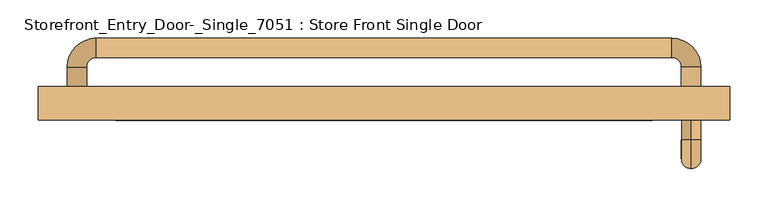
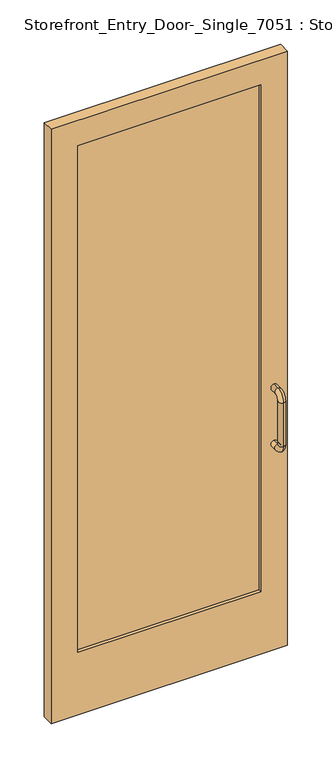
"""IFC4 building model written with IfcOpenShell, lengths in millimetres: door geometry, Storefront_Entry_Door-_Single_7051 : Store Front Single Door."""

import ifcopenshell
import ifcopenshell.guid

model = None  # the IFC model being written
_history = None  # IfcOwnerHistory: only IFC2X3 demands one
_inside = {}  # id of a spatial element -> (the spatial element, [elements in it])
_under = {}  # id of a project, library or spatial element -> (it, [spatial elements below it])
_declared = {}  # id of a project -> (the project, [libraries it declares])
_typed = {}  # id of a type object -> (the type object, [elements of that type])
_made_of = {}  # id of a material, layer set ... -> (it, [elements and type objects made of it])


def new_model(schema):
    """Start an empty IFC model of exactly this schema.

    Asked for "IFC4X3", IfcOpenShell would pick the latest addendum, in which some entities
    have other attributes; the version numbers below select the first issue.
    IFC2X3 requires an IfcOwnerHistory on every rooted entity: one is made here for all.
    """
    global model, _history
    if schema == "IFC4X3":
        model = ifcopenshell.file(schema_version=(4, 3, 0, 0))
    else:
        model = ifcopenshell.file(schema=schema)
    _inside.clear()
    _under.clear()
    _declared.clear()
    _typed.clear()
    _made_of.clear()
    _history = None
    if model.schema == "IFC2X3":
        org = make("IfcOrganization", Name="unknown")
        user = make(
            "IfcPersonAndOrganization",
            ThePerson=make("IfcPerson", FamilyName="unknown"),
            TheOrganization=org,
        )
        app = make(
            "IfcApplication",
            ApplicationDeveloper=org,
            Version="unknown",
            ApplicationFullName="unknown",
            ApplicationIdentifier="unknown",
        )
        _history = make(
            "IfcOwnerHistory",
            OwningUser=user,
            OwningApplication=app,
            ChangeAction="ADDED",
            CreationDate=0,
        )
    return model


def make(cls, **values):
    """One entity of the class cls with the attributes given. An attribute that is None is left unset."""
    return model.create_entity(
        cls, **{name: value for name, value in values.items() if value is not None}
    )


def rooted(cls, **values):
    """An entity with a GlobalId (a new one), such as an element, a storey or a relation."""
    return make(cls, GlobalId=ifcopenshell.guid.new(), OwnerHistory=_history, **values)


def si_unit(unit_type, name, prefix=None):
    """IfcSIUnit, for example si_unit("LENGTHUNIT", "METRE", prefix="MILLI")."""
    return make("IfcSIUnit", UnitType=unit_type, Prefix=prefix, Name=name)


def assignment(units):
    """IfcUnitAssignment: the units of a project."""
    return None if units is None else make("IfcUnitAssignment", Units=units)


def point(xyz):
    """IfcCartesianPoint."""
    return None if xyz is None else make("IfcCartesianPoint", Coordinates=xyz)


def direction(xyz):
    """IfcDirection."""
    return None if xyz is None else make("IfcDirection", DirectionRatios=xyz)


def frame(location, z_axis=None, x_axis=None):
    """IfcAxis2Placement3D, a coordinate frame: its origin and axes. An axis left out is left unset."""
    return make(
        "IfcAxis2Placement3D",
        Location=point(location),
        Axis=direction(z_axis),
        RefDirection=direction(x_axis),
    )


def origin():
    """The frame at (0, 0, 0) with its axes left unset."""
    return frame((0.0, 0.0, 0.0))


def place(relative_to, where):
    """IfcLocalPlacement: puts the frame where relative to a parent placement (None: the world)."""
    return make(
        "IfcLocalPlacement", PlacementRelTo=relative_to, RelativePlacement=where
    )


def context(
    kind, dimensions, precision=None, world=None, true_north=None, identifier=None
):
    """IfcGeometricRepresentationContext, for example the 3D "Model" context."""
    return make(
        "IfcGeometricRepresentationContext",
        ContextIdentifier=identifier,
        ContextType=kind,
        CoordinateSpaceDimension=dimensions,
        Precision=precision,
        WorldCoordinateSystem=world,
        TrueNorth=true_north,
    )


def project(units=None, contexts=None):
    """IfcProject with its units and contexts."""
    return rooted(
        "IfcProject",
        Name="project",
        RepresentationContexts=contexts,
        UnitsInContext=assignment(units),
    )


def spatial(cls, under=None, at=None, **own):
    """A site, building, storey or space (cls), placed at a placement, below another one or the project."""
    s = rooted(cls, ObjectPlacement=at, **own)
    if under is not None:
        _under.setdefault(under.id(), (under, []))[1].append(s)
    return s


def polyline(points):
    """IfcPolyline through the points."""
    return make("IfcPolyline", Points=[point(p) for p in points])


def circle_curve(where, radius):
    """IfcCircle in the frame where."""
    return make("IfcCircle", Position=where, Radius=radius)


def ellipse_curve(where, semi_axis1, semi_axis2):
    """IfcEllipse in the frame where."""
    return make(
        "IfcEllipse", Position=where, SemiAxis1=semi_axis1, SemiAxis2=semi_axis2
    )


def trimmed(basis, trim1, trim2, sense, master):
    """IfcTrimmedCurve: the piece of a basis curve between two trims."""
    return make(
        "IfcTrimmedCurve",
        BasisCurve=basis,
        Trim1=trim1,
        Trim2=trim2,
        SenseAgreement=sense,
        MasterRepresentation=master,
    )


def outline(outer, holes=None, kind="AREA"):
    """IfcArbitraryClosedProfileDef: a profile drawn as a closed curve; with holes, ...WithVoids."""
    if holes is None:
        return make("IfcArbitraryClosedProfileDef", ProfileType=kind, OuterCurve=outer)
    return make(
        "IfcArbitraryProfileDefWithVoids",
        ProfileType=kind,
        OuterCurve=outer,
        InnerCurves=holes,
    )


def extrude(swept, where, along, depth):
    """IfcExtrudedAreaSolid: the profile swept, set in the frame where, extruded along a direction by depth."""
    return make(
        "IfcExtrudedAreaSolid",
        SweptArea=swept,
        Position=where,
        ExtrudedDirection=direction(along),
        Depth=depth,
    )


def shape(context_of_items, identifier, shape_type, items):
    """IfcShapeRepresentation: the items that make up one representation, for example the "Body"."""
    return make(
        "IfcShapeRepresentation",
        ContextOfItems=context_of_items,
        RepresentationIdentifier=identifier,
        RepresentationType=shape_type,
        Items=items,
    )


def source(mapping_origin, context_of_items, identifier, shape_type, items):
    """IfcRepresentationMap: a shape defined once, which mapped items show again and again."""
    return make(
        "IfcRepresentationMap",
        MappingOrigin=mapping_origin,
        MappedRepresentation=shape(context_of_items, identifier, shape_type, items),
    )


def transform(
    local_origin,
    x_axis=None,
    y_axis=None,
    z_axis=None,
    scale=None,
    scale2=None,
    scale3=None,
    uniform=True,
):
    """IfcCartesianTransformationOperator3D, or its non-uniform kind. x_axis, y_axis, z_axis: its Axis1, 2, 3."""
    if uniform:
        return make(
            "IfcCartesianTransformationOperator3D",
            Axis1=direction(x_axis),
            Axis2=direction(y_axis),
            LocalOrigin=point(local_origin),
            Scale=scale,
            Axis3=direction(z_axis),
        )
    return make(
        "IfcCartesianTransformationOperator3DnonUniform",
        Axis1=direction(x_axis),
        Axis2=direction(y_axis),
        LocalOrigin=point(local_origin),
        Scale=scale,
        Axis3=direction(z_axis),
        Scale2=scale2,
        Scale3=scale3,
    )


def mapped(mapping_source, mapping_target):
    """IfcMappedItem: shows the shape of a source again, moved by a transform."""
    return make(
        "IfcMappedItem", MappingSource=mapping_source, MappingTarget=mapping_target
    )


def made_of(thing, what):
    """Note that an element or type object is made of a material, layer set ...; save() writes the relation."""
    if what is not None:
        _made_of.setdefault(what.id(), (what, []))[1].append(thing)
    return thing


def element(
    cls,
    number,
    at=None,
    inside=None,
    cuts=None,
    type_object=None,
    material=None,
    context=None,
    identifier="Body",
    shape_type=None,
    held_by="IfcProductDefinitionShape",
    body=None,
    shapes=None,
    **own,
):
    """One element of the class cls, such as IfcWall. Its Tag is "e" and its number.

    at: its placement. inside: the storey or other place that contains it. cuts: it is an
    opening in that element (IfcRelVoidsElement). A single representation is given by context,
    identifier, shape_type and body (its items); several are given by shapes. held_by: the class
    of the entity that holds the representations. save() writes the other relations.
    """
    e = rooted(cls, Tag="e%d" % number, ObjectPlacement=at, **own)
    if body is not None:
        shapes = [shape(context, identifier, shape_type, body)]
    if shapes is not None:
        e.Representation = make(held_by, Representations=shapes)
    if inside is not None:
        _inside.setdefault(inside.id(), (inside, []))[1].append(e)
    if cuts is not None:
        rooted(
            "IfcRelVoidsElement", RelatingBuildingElement=cuts, RelatedOpeningElement=e
        )
    if type_object is not None:
        _typed.setdefault(type_object.id(), (type_object, []))[1].append(e)
    return made_of(e, material)


def aggregate(whole, parts):
    """IfcRelAggregates: a whole, such as a stair, and the parts it consists of."""
    return rooted("IfcRelAggregates", RelatingObject=whole, RelatedObjects=parts)


def save(model, path):
    """Write the relations noted so far, then the file.

    IfcRelAggregates (storeys below a building ...), IfcRelContainedInSpatialStructure (elements
    in a storey), IfcRelDefinesByType, IfcRelAssociatesMaterial and IfcRelDeclares: one each for
    every whole, place, type object, material and project.
    """
    for whole, parts in _under.values():
        aggregate(whole, parts)
    for where, things in _inside.values():
        rooted(
            "IfcRelContainedInSpatialStructure",
            RelatedElements=things,
            RelatingStructure=where,
        )
    for kind, things in _typed.values():
        rooted("IfcRelDefinesByType", RelatedObjects=things, RelatingType=kind)
    for what, things in _made_of.values():
        rooted("IfcRelAssociatesMaterial", RelatedObjects=things, RelatingMaterial=what)
    for by, libraries in _declared.values():
        rooted("IfcRelDeclares", RelatingContext=by, RelatedDefinitions=libraries)
    model.write(path)


def plane_surface(at):
    """IfcPlane: the flat surface through the origin of the frame at, square to its z axis."""
    return make("IfcPlane", Position=at)


def cylinder_surface(at, radius):
    """IfcCylindricalSurface: all points at the distance radius from the z axis of the frame at."""
    return make("IfcCylindricalSurface", Position=at, Radius=radius)


def revolved_surface(curve, axis_point, axis_direction):
    """IfcSurfaceOfRevolution: the curve turned about the line through axis_point along axis_direction."""
    return make(
        "IfcSurfaceOfRevolution",
        SweptCurve=make("IfcArbitraryOpenProfileDef", ProfileType="CURVE", Curve=curve),
        AxisPosition=make("IfcAxis1Placement", Location=point(axis_point), Axis=direction(axis_direction)),
    )


def advanced_brep(points, edges, surfaces, faces):
    """IfcAdvancedBrep: a solid bounded by faces that lie on surfaces and meet in shared edges.

    An edge is (start, end): straight between two places in points (the first is 0);
    or (start, end, curve); or (start, end, curve, False) where it runs against its curve.
    A face is (place in surfaces, loops), or (place, loops, False) where it looks against
    its surface's normal. A loop lists edges by number (the first is 1), with a minus sign
    where the edge is run from its end to its start. The first loop is the outer one.
    """
    corners = [point(p) for p in points]
    vertices = [make("IfcVertexPoint", VertexGeometry=c) for c in corners]
    made = []
    for start, end, *more in edges:
        made.append(
            make(
                "IfcEdgeCurve",
                EdgeStart=vertices[start],
                EdgeEnd=vertices[end],
                EdgeGeometry=more[0] if more else make("IfcPolyline", Points=[corners[start], corners[end]]),
                SameSense=more[1] if len(more) > 1 else True,
            )
        )
    hull = []
    for where, loops, *sense in faces:
        bounds = []
        for j, loop in enumerate(loops):
            ring = [make("IfcOrientedEdge", EdgeElement=made[abs(k) - 1], Orientation=k > 0) for k in loop]
            bounds.append(
                make(
                    "IfcFaceOuterBound" if j == 0 else "IfcFaceBound",
                    Bound=make("IfcEdgeLoop", EdgeList=ring),
                    Orientation=True,
                )
            )
        hull.append(make("IfcAdvancedFace", Bounds=bounds, FaceSurface=surfaces[where], SameSense=sense[0] if sense else True))
    return make("IfcAdvancedBrep", Outer=make("IfcClosedShell", CfsFaces=hull))


def storefront_entry_door_single_7051_store_front_single_door_ff742114(model_context):
    return source(origin(), model_context, "Body", "SolidModel", [
        advanced_brep(
        [(402.7714285, -50.8, 1054.1), (402.7714285, -50.8, 1079.5), (402.7714285, -76.2, 1079.5), (402.7714285, -76.2, 1054.1), (402.7714285, -114.3, 1041.4), (402.7714285, -88.9, 1041.4), (402.7714285, -114.3, 863.6), (402.7714285, -88.9, 863.6), (402.7714285, -76.2, 825.5), (402.7714285, -76.2, 850.9), (402.7714285, -50.8, 850.9), (402.7714285, -50.8, 825.5)],
        [
            (0, 1, circle_curve(frame((402.7714285, -50.8, 1066.8), z_axis=(0.0, 1.0, 0.0), x_axis=(0.0, 0.0, 1.0)), 12.7)),
            (1, 0, circle_curve(frame((402.7714285, -50.8, 1066.8), z_axis=(0.0, 1.0, 0.0), x_axis=(0.0, 0.0, 1.0)), 12.7)),
            (1, 2),
            (2, 3, circle_curve(frame((402.7714285, -76.2, 1066.8), z_axis=(0.0, 1.0, 0.0), x_axis=(0.0, 0.0, 1.0)), 12.7)),
            (3, 0),
            (3, 2, circle_curve(frame((402.7714285, -76.2, 1066.8), z_axis=(0.0, 1.0, 0.0), x_axis=(0.0, 0.0, 1.0)), 12.7)),
            (4, 5, circle_curve(frame((402.7714285, -101.6, 1041.4), z_axis=(0.0, 0.0, 1.0), x_axis=(0.0, -1.0, 0.0)), 12.7)),
            (5, 3, circle_curve(frame((402.7714285, -76.2, 1041.4), z_axis=(-1.0, 0.0, 0.0), x_axis=(0.0, 0.0, 1.0)), 12.7)),
            (2, 4, circle_curve(frame((402.7714285, -76.2, 1041.4), z_axis=(1.0, 0.0, 0.0), x_axis=(0.0, 0.0, 1.0)), 38.1)),
            (5, 4, circle_curve(frame((402.7714285, -101.6, 1041.4), z_axis=(0.0, 0.0, 1.0), x_axis=(0.0, -1.0, 0.0)), 12.7)),
            (4, 6),
            (6, 7, circle_curve(frame((402.7714285, -101.6, 863.6), z_axis=(0.0, 0.0, 1.0), x_axis=(0.0, -1.0, 0.0)), 12.7)),
            (7, 5),
            (7, 6, circle_curve(frame((402.7714285, -101.6, 863.6), z_axis=(0.0, 0.0, 1.0), x_axis=(0.0, -1.0, 0.0)), 12.7)),
            (8, 9, circle_curve(frame((402.7714285, -76.2, 838.2), z_axis=(0.0, -1.0, 0.0), x_axis=(0.0, 0.0, -1.0)), 12.7)),
            (9, 7, circle_curve(frame((402.7714285, -76.2, 863.6), z_axis=(-1.0, 0.0, 0.0), x_axis=(0.0, -1.0, 0.0)), 12.7)),
            (6, 8, circle_curve(frame((402.7714285, -76.2, 863.6), z_axis=(1.0, 0.0, 0.0), x_axis=(0.0, -1.0, 0.0)), 38.1)),
            (9, 8, circle_curve(frame((402.7714285, -76.2, 838.2), z_axis=(0.0, -1.0, 0.0), x_axis=(0.0, 0.0, -1.0)), 12.7)),
            (10, 11, circle_curve(frame((402.7714285, -50.8, 838.2), z_axis=(0.0, 1.0, 0.0), x_axis=(0.0, 0.0, -1.0)), 12.7)),
            (11, 10, circle_curve(frame((402.7714285, -50.8, 838.2), z_axis=(0.0, 1.0, 0.0), x_axis=(0.0, 0.0, -1.0)), 12.7)),
            (8, 11),
            (10, 9),
        ],
        [
            plane_surface(frame((402.7714285, -50.8, 1066.8), z_axis=(0.0, 1.0, 0.0), x_axis=(1.0, 0.0, 0.0))),
            cylinder_surface(frame((402.7714285, -50.8, 1066.8), z_axis=(0.0, 1.0, 0.0), x_axis=(0.0, 0.0, 1.0)), 12.7),
            revolved_surface(trimmed(ellipse_curve(frame((402.7714285, -76.2, 1066.8), z_axis=(0.0, -1.0, 0.0), x_axis=(0.0, 0.0, 1.0)), 12.7, 12.7), [point((402.7714285, -76.2, 1054.1))], [point((402.7714285, -76.2, 1079.5))], True, "CARTESIAN"), (402.7714285, -76.2, 1041.4), (-1.0, 0.0, 0.0)),
            revolved_surface(trimmed(ellipse_curve(frame((402.7714285, -76.2, 1066.8), z_axis=(0.0, -1.0, 0.0), x_axis=(0.0, 0.0, 1.0)), 12.7, 12.7), [point((402.7714285, -76.2, 1079.5))], [point((402.7714285, -76.2, 1054.1))], True, "CARTESIAN"), (402.7714285, -76.2, 1041.4), (-1.0, 0.0, 0.0)),
            cylinder_surface(frame((402.7714285, -101.6, 1041.4), z_axis=(0.0, 0.0, 1.0), x_axis=(0.0, -1.0, 0.0)), 12.7),
            revolved_surface(trimmed(ellipse_curve(frame((402.7714285, -101.6, 863.6), z_axis=(0.0, 0.0, -1.0), x_axis=(0.0, -1.0, 0.0)), 12.7, 12.7), [point((402.7714285, -88.9, 863.6))], [point((402.7714285, -114.3, 863.6))], True, "CARTESIAN"), (402.7714285, -76.2, 863.6), (-1.0, 0.0, 0.0)),
            revolved_surface(trimmed(ellipse_curve(frame((402.7714285, -101.6, 863.6), z_axis=(0.0, 0.0, -1.0), x_axis=(0.0, -1.0, 0.0)), 12.7, 12.7), [point((402.7714285, -114.3, 863.6))], [point((402.7714285, -88.9, 863.6))], True, "CARTESIAN"), (402.7714285, -76.2, 863.6), (-1.0, 0.0, 0.0)),
            plane_surface(frame((402.7714285, -50.8, 838.2), z_axis=(0.0, 1.0, 0.0), x_axis=(1.0, 0.0, 0.0))),
            cylinder_surface(frame((402.7714285, -76.2, 838.2), z_axis=(0.0, -1.0, 0.0), x_axis=(0.0, 0.0, -1.0)), 12.7),
        ],
        [
            (0, [[1, 2]]),
            (1, [[3, 4, 5, -2]]),
            (1, [[-5, 6, -3, -1]]),
            (2, [[7, 8, -4, 9]]),
            (3, [[10, -9, -6, -8]]),
            (4, [[11, 12, 13, -7]]),
            (4, [[-13, 14, -11, -10]]),
            (5, [[15, 16, -12, 17]]),
            (6, [[18, -17, -14, -16]]),
            (7, [[19, 20]]),
            (8, [[21, -19, 22, -15]]),
            (8, [[-22, -20, -21, -18]]),
        ],
    ),
        advanced_brep(
        [(390.0714285, -6.35, 1066.8), (415.4714285, -6.35, 1066.8), (415.4714285, 19.05, 1066.8), (390.0714285, 19.05, 1066.8), (377.3714285, 57.15, 1066.8), (377.3714285, 31.75, 1066.8), (-377.3714285, 57.15, 1066.8), (-377.3714285, 31.75, 1066.8), (-415.4714285, 19.05, 1066.8), (-390.0714285, 19.05, 1066.8), (-390.0714285, -6.35, 1066.8), (-415.4714285, -6.35, 1066.8)],
        [
            (0, 1, circle_curve(frame((402.7714285, -6.35, 1066.8), z_axis=(0.0, -1.0, 0.0), x_axis=(1.0, 0.0, 0.0)), 12.7)),
            (1, 0, circle_curve(frame((402.7714285, -6.35, 1066.8), z_axis=(0.0, -1.0, 0.0), x_axis=(1.0, 0.0, 0.0)), 12.7)),
            (1, 2),
            (2, 3, circle_curve(frame((402.7714285, 19.05, 1066.8), z_axis=(0.0, -1.0, 0.0), x_axis=(1.0, 0.0, 0.0)), 12.7)),
            (3, 0),
            (3, 2, circle_curve(frame((402.7714285, 19.05, 1066.8), z_axis=(0.0, -1.0, 0.0), x_axis=(1.0, 0.0, 0.0)), 12.7)),
            (4, 5, circle_curve(frame((377.3714285, 44.45, 1066.8), z_axis=(1.0, 0.0, 0.0), x_axis=(0.0, 1.0, 0.0)), 12.7)),
            (5, 3, circle_curve(frame((377.3714285, 19.05, 1066.8), z_axis=(0.0, 0.0, -1.0), x_axis=(1.0, 0.0, 0.0)), 12.7)),
            (2, 4, circle_curve(frame((377.3714285, 19.05, 1066.8), z_axis=(0.0, 0.0, 1.0), x_axis=(1.0, 0.0, 0.0)), 38.1)),
            (5, 4, circle_curve(frame((377.3714285, 44.45, 1066.8), z_axis=(1.0, 0.0, 0.0), x_axis=(0.0, 1.0, 0.0)), 12.7)),
            (4, 6),
            (6, 7, circle_curve(frame((-377.3714285, 44.45, 1066.8), z_axis=(1.0, 0.0, 0.0), x_axis=(0.0, 1.0, 0.0)), 12.7)),
            (7, 5),
            (7, 6, circle_curve(frame((-377.3714285, 44.45, 1066.8), z_axis=(1.0, 0.0, 0.0), x_axis=(0.0, 1.0, 0.0)), 12.7)),
            (8, 9, circle_curve(frame((-402.7714285, 19.05, 1066.8), z_axis=(0.0, 1.0, 0.0), x_axis=(-1.0, 0.0, 0.0)), 12.7)),
            (9, 7, circle_curve(frame((-377.3714285, 19.05, 1066.8), z_axis=(0.0, 0.0, -1.0), x_axis=(0.0, 1.0, 0.0)), 12.7)),
            (6, 8, circle_curve(frame((-377.3714285, 19.05, 1066.8), z_axis=(0.0, 0.0, 1.0), x_axis=(0.0, 1.0, 0.0)), 38.1)),
            (9, 8, circle_curve(frame((-402.7714285, 19.05, 1066.8), z_axis=(0.0, 1.0, 0.0), x_axis=(-1.0, 0.0, 0.0)), 12.7)),
            (10, 11, circle_curve(frame((-402.7714285, -6.35, 1066.8), z_axis=(0.0, -1.0, 0.0), x_axis=(-1.0, 0.0, 0.0)), 12.7)),
            (11, 10, circle_curve(frame((-402.7714285, -6.35, 1066.8), z_axis=(0.0, -1.0, 0.0), x_axis=(-1.0, 0.0, 0.0)), 12.7)),
            (8, 11),
            (10, 9),
        ],
        [
            plane_surface(frame((402.7714285, -6.35, 1066.8), z_axis=(0.0, -1.0, 0.0), x_axis=(0.0, 0.0, 1.0))),
            cylinder_surface(frame((402.7714285, -6.35, 1066.8), z_axis=(0.0, -1.0, 0.0), x_axis=(1.0, 0.0, 0.0)), 12.7),
            revolved_surface(trimmed(ellipse_curve(frame((402.7714285, 19.05, 1066.8), z_axis=(0.0, 1.0, 0.0), x_axis=(1.0, 0.0, 0.0)), 12.7, 12.7), [point((390.0714285, 19.05, 1066.8))], [point((415.4714285, 19.05, 1066.8))], True, "CARTESIAN"), (377.3714285, 19.05, 1066.8), (0.0, 0.0, -1.0)),
            revolved_surface(trimmed(ellipse_curve(frame((402.7714285, 19.05, 1066.8), z_axis=(0.0, 1.0, 0.0), x_axis=(1.0, 0.0, 0.0)), 12.7, 12.7), [point((415.4714285, 19.05, 1066.8))], [point((390.0714285, 19.05, 1066.8))], True, "CARTESIAN"), (377.3714285, 19.05, 1066.8), (0.0, 0.0, -1.0)),
            cylinder_surface(frame((377.3714285, 44.45, 1066.8), z_axis=(1.0, 0.0, 0.0), x_axis=(0.0, 1.0, 0.0)), 12.7),
            revolved_surface(trimmed(ellipse_curve(frame((-377.3714285, 44.45, 1066.8), z_axis=(-1.0, 0.0, 0.0), x_axis=(0.0, 1.0, 0.0)), 12.7, 12.7), [point((-377.3714285, 31.75, 1066.8))], [point((-377.3714285, 57.15, 1066.8))], True, "CARTESIAN"), (-377.3714285, 19.05, 1066.8), (0.0, 0.0, -1.0)),
            revolved_surface(trimmed(ellipse_curve(frame((-377.3714285, 44.45, 1066.8), z_axis=(-1.0, 0.0, 0.0), x_axis=(0.0, 1.0, 0.0)), 12.7, 12.7), [point((-377.3714285, 57.15, 1066.8))], [point((-377.3714285, 31.75, 1066.8))], True, "CARTESIAN"), (-377.3714285, 19.05, 1066.8), (0.0, 0.0, -1.0)),
            plane_surface(frame((-402.7714285, -6.35, 1066.8), z_axis=(0.0, -1.0, 0.0), x_axis=(0.0, 0.0, 1.0))),
            cylinder_surface(frame((-402.7714285, 19.05, 1066.8), z_axis=(0.0, 1.0, 0.0), x_axis=(-1.0, 0.0, 0.0)), 12.7),
        ],
        [
            (0, [[1, 2]]),
            (1, [[3, 4, 5, -2]]),
            (1, [[-5, 6, -3, -1]]),
            (2, [[7, 8, -4, 9]]),
            (3, [[10, -9, -6, -8]]),
            (4, [[11, 12, 13, -7]]),
            (4, [[-13, 14, -11, -10]]),
            (5, [[15, 16, -12, 17]]),
            (6, [[18, -17, -14, -16]]),
            (7, [[19, 20]]),
            (8, [[21, -19, 22, -15]]),
            (8, [[-22, -20, -21, -18]]),
        ],
    ),
        extrude(outline(polyline([(351.9714285, -19.05), (351.9714285, -38.1), (-351.9714285, -38.1), (-351.9714285, -19.05), (351.9714285, -19.05)])), frame((0.0, 0.0, 254.0), z_axis=(0.0, 0.0, 1.0), x_axis=(1.0, 0.0, 0.0)), (0.0, 0.0, 1.0), 2057.4),
        extrude(outline(polyline([(2413.0, 453.5714285), (2413.0, -453.5714285), (0.0, -453.5714285), (0.0, 453.5714285), (2413.0, 453.5714285)]), holes=[polyline([(2311.4, -351.9714285), (2311.4, 351.9714285), (254.0, 351.9714285), (254.0, -351.9714285), (2311.4, -351.9714285)])]), frame((0.0, -50.8, 0.0), z_axis=(0.0, 1.0, 0.0), x_axis=(0.0, 0.0, 1.0)), (0.0, 0.0, 1.0), 44.45),
    ])


if __name__ == "__main__":
    model = new_model("IFC4")
    model_context = context("Model", 3, world=origin())
    ifc_project = project(units=[si_unit("LENGTHUNIT", "METRE", prefix="MILLI")], contexts=[model_context])
    site = spatial("IfcSite", under=ifc_project)
    building = spatial("IfcBuilding", under=site)
    placement = place(None, origin())
    storefront_entry_door_single_7051_store_front_single_door_shape = storefront_entry_door_single_7051_store_front_single_door_ff742114(model_context)
    element("IfcDoor", 1, ObjectType="Storefront_Entry_Door-_Single_7051 : Store Front Single Door", at=placement, inside=building, context=model_context, shape_type="MappedRepresentation", body=[
        mapped(storefront_entry_door_single_7051_store_front_single_door_shape, transform((0.0, 0.0, 0.0), x_axis=(1.0, 0.0, 0.0), y_axis=(0.0, 1.0, 0.0), z_axis=(0.0, 0.0, 1.0))),
    ])
    save(model, "model.ifc")

# Revit data of these elements
# Type "Storefront_Entry_Door-_Single_7051 : Store Front Single Door"
#   Type Mark = "19"
#   Assembly Code = "B2030110"
#   Analytic Construction = "<None>"
#   Top Rail = 0' - 4"
#   Side Rail = 0' - 4"
#   Reporting Width [instance default] = 4' - 2"
#   Rail Height AFF = 3' - 6"
#   Offset = 0' - 2"
#   Door Width [instance default] = 4' - 2"
#   Bottom Rail Width = 0' - 10"
#   Material = Metal - Aluminum
#   Glazing Material = Glass
#   Function = (empty or 0)
# Element 1 (IfcDoor, "Storefront_Entry_Door-_Single_7051 : Store Front Single Door")
#   Reporting Width = 2' - 11.71429"
#   Door Width = 2' - 11.71429"
#   Materials on its faces: "Metal - Aluminum", "Glass"
# Materials
#   "Metal - Aluminum": class "Metal", colour RGB 247 247 247, transparency 0
#   "Glass": class "Glass", colour RGB 218 227 224, transparency 0.85, Description = "Soda Lime Glass", Cost = 0
